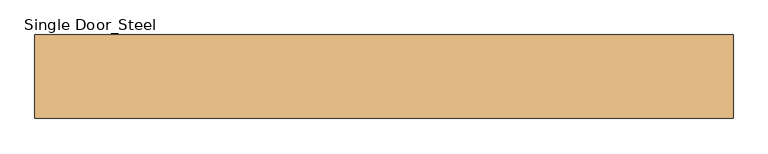
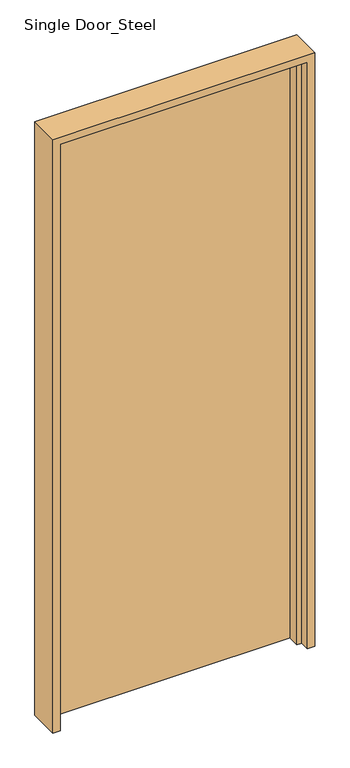
"""IFC4 building model written with IfcOpenShell, lengths in millimetres: door geometry, Single Door_Steel : H_DR_AR B12_Door_Single_W1100xH2580_No FR_SD-6."""

from ifc_helpers import new_model, si_unit, origin, origin_with_axes, place, context, project, spatial, polyline, outline, extrude, faceted_brep, source, transform, mapped, element, save


def single_door_steel_57e6a368(model_context):
    return source(origin(), model_context, "Body", "SolidModel", [
        extrude(outline(polyline([(505.0, 64.0), (505.0, 24.0), (-505.0, 24.0), (-505.0, 64.0), (505.0, 64.0)])), origin_with_axes(), (0.0, 0.0, 1.0), 2535.0),
        faceted_brep([(505.0, 64.0, 0.0), (535.0, 64.0, 0.0), (535.0, -64.0, 0.0), (505.0, -64.0, 0.0), (505.0, -24.0, 0.0), (485.0, -24.0, 0.0), (485.0, 24.0, 0.0), (505.0, 24.0, 0.0), (-505.0, 64.0, 0.0), (-505.0, 24.0, 0.0), (-485.0, 24.0, 0.0), (-485.0, -24.0, 0.0), (-505.0, -24.0, 0.0), (-505.0, -64.0, 0.0), (-535.0, -64.0, 0.0), (-535.0, 64.0, 0.0), (505.0, 64.0, 2535.0), (-505.0, 64.0, 2535.0), (-535.0, 64.0, 2565.0), (535.0, 64.0, 2565.0), (535.0, -64.0, 2565.0), (-535.0, -64.0, 2565.0), (-505.0, -64.0, 2535.0), (505.0, -64.0, 2535.0), (505.0, -24.0, 2535.0), (-505.0, -24.0, 2535.0), (-485.0, -24.0, 2515.0), (485.0, -24.0, 2515.0), (485.0, 24.0, 2515.0), (-485.0, 24.0, 2515.0), (-505.0, 24.0, 2535.0), (505.0, 24.0, 2535.0)], [[[0, 1, 2, 3, 4, 5, 6, 7]], [[8, 9, 10, 11, 12, 13, 14, 15]], [[1, 0, 16, 17, 8, 15, 18, 19]], [[2, 1, 19, 20]], [[3, 2, 20, 21, 14, 13, 22, 23]], [[4, 3, 23, 24]], [[5, 4, 24, 25, 12, 11, 26, 27]], [[6, 5, 27, 28]], [[7, 6, 28, 29, 10, 9, 30, 31]], [[0, 7, 31, 16]], [[17, 30, 9, 8]], [[21, 18, 15, 14]], [[25, 22, 13, 12]], [[29, 26, 11, 10]], [[16, 31, 30, 17]], [[20, 19, 18, 21]], [[24, 23, 22, 25]], [[28, 27, 26, 29]]]),
    ])


if __name__ == "__main__":
    model = new_model("IFC4")
    model_context = context("Model", 3, world=origin())
    ifc_project = project(units=[si_unit("LENGTHUNIT", "METRE", prefix="MILLI")], contexts=[model_context])
    site = spatial("IfcSite", under=ifc_project)
    building = spatial("IfcBuilding", under=site)
    placement = place(None, origin())
    single_door_steel_shape = single_door_steel_57e6a368(model_context)
    element("IfcDoor", 1, ObjectType="Single Door_Steel : H_DR_AR B12_Door_Single_W1100xH2580_No FR_SD-6", at=placement, inside=building, context=model_context, shape_type="MappedRepresentation", body=[
        mapped(single_door_steel_shape, transform((0.0, 0.0, 0.0), x_axis=(1.0, 0.0, 0.0), y_axis=(0.0, 1.0, 0.0), z_axis=(0.0, 0.0, 1.0))),
    ])
    save(model, "model.ifc")

# Revit data of these elements
# Type "Single Door_Steel : H_DR_AR B12_Door_Single_W1100xH2580_No FR_SD-6"
#   Type Mark = "436"
#   Analytic Construction = "<None>"
#   프레임 투영 외부. = 25 mm
#   프레임 투영 내부. = 25 mm
#   프레임 폭 = 75 mm
#   Height = 2580 mm
#   Width = 1100 mm
#   Define Thermal Properties by = 1
#   문 패널 = none
#   문 프레임 = none
#   Function = (empty or 0)
#   Wall Closure = (empty or 0)
